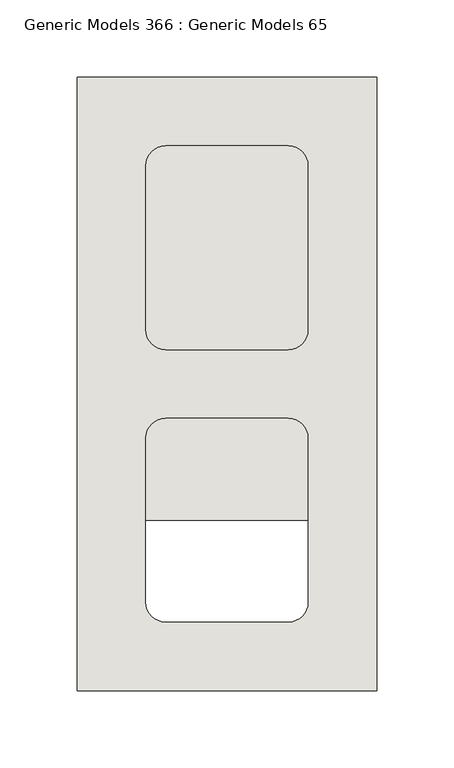
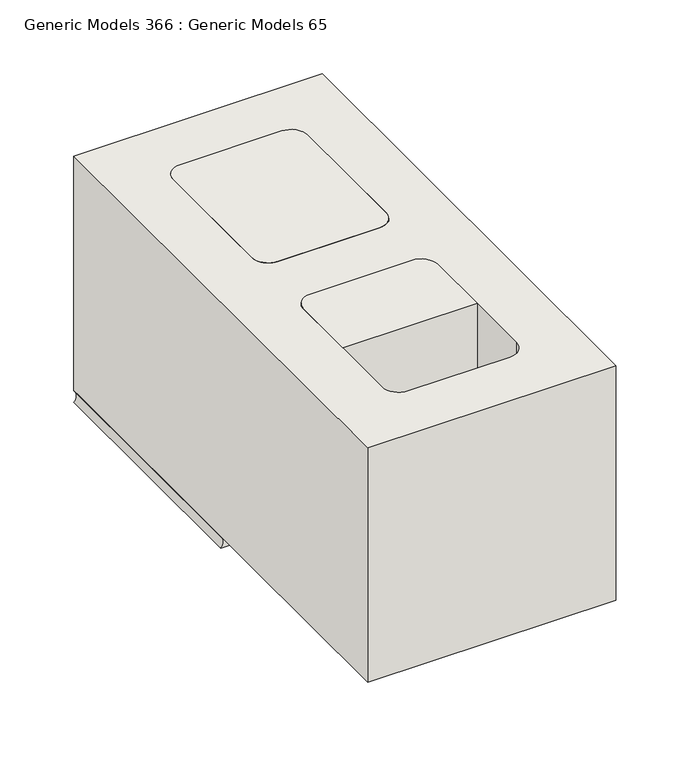
"""IFC4 building model written with IfcOpenShell, lengths in millimetres: wall geometry, Generic Models 366 : Generic Models 65."""

import ifcopenshell
import ifcopenshell.guid

model = None  # the IFC model being written
_history = None  # IfcOwnerHistory: only IFC2X3 demands one
_inside = {}  # id of a spatial element -> (the spatial element, [elements in it])
_under = {}  # id of a project, library or spatial element -> (it, [spatial elements below it])
_declared = {}  # id of a project -> (the project, [libraries it declares])
_typed = {}  # id of a type object -> (the type object, [elements of that type])
_made_of = {}  # id of a material, layer set ... -> (it, [elements and type objects made of it])


def new_model(schema):
    """Start an empty IFC model of exactly this schema.

    Asked for "IFC4X3", IfcOpenShell would pick the latest addendum, in which some entities
    have other attributes; the version numbers below select the first issue.
    IFC2X3 requires an IfcOwnerHistory on every rooted entity: one is made here for all.
    """
    global model, _history
    if schema == "IFC4X3":
        model = ifcopenshell.file(schema_version=(4, 3, 0, 0))
    else:
        model = ifcopenshell.file(schema=schema)
    _inside.clear()
    _under.clear()
    _declared.clear()
    _typed.clear()
    _made_of.clear()
    _history = None
    if model.schema == "IFC2X3":
        org = make("IfcOrganization", Name="unknown")
        user = make(
            "IfcPersonAndOrganization",
            ThePerson=make("IfcPerson", FamilyName="unknown"),
            TheOrganization=org,
        )
        app = make(
            "IfcApplication",
            ApplicationDeveloper=org,
            Version="unknown",
            ApplicationFullName="unknown",
            ApplicationIdentifier="unknown",
        )
        _history = make(
            "IfcOwnerHistory",
            OwningUser=user,
            OwningApplication=app,
            ChangeAction="ADDED",
            CreationDate=0,
        )
    return model


def make(cls, **values):
    """One entity of the class cls with the attributes given. An attribute that is None is left unset."""
    return model.create_entity(
        cls, **{name: value for name, value in values.items() if value is not None}
    )


def rooted(cls, **values):
    """An entity with a GlobalId (a new one), such as an element, a storey or a relation."""
    return make(cls, GlobalId=ifcopenshell.guid.new(), OwnerHistory=_history, **values)


def si_unit(unit_type, name, prefix=None):
    """IfcSIUnit, for example si_unit("LENGTHUNIT", "METRE", prefix="MILLI")."""
    return make("IfcSIUnit", UnitType=unit_type, Prefix=prefix, Name=name)


def assignment(units):
    """IfcUnitAssignment: the units of a project."""
    return None if units is None else make("IfcUnitAssignment", Units=units)


def point(xyz):
    """IfcCartesianPoint."""
    return None if xyz is None else make("IfcCartesianPoint", Coordinates=xyz)


def direction(xyz):
    """IfcDirection."""
    return None if xyz is None else make("IfcDirection", DirectionRatios=xyz)


def frame(location, z_axis=None, x_axis=None):
    """IfcAxis2Placement3D, a coordinate frame: its origin and axes. An axis left out is left unset."""
    return make(
        "IfcAxis2Placement3D",
        Location=point(location),
        Axis=direction(z_axis),
        RefDirection=direction(x_axis),
    )


def frame_2d(location, x_axis=None):
    """IfcAxis2Placement2D, a coordinate frame in the plane: its origin and x axis."""
    return make(
        "IfcAxis2Placement2D", Location=point(location), RefDirection=direction(x_axis)
    )


def origin():
    """The frame at (0, 0, 0) with its axes left unset."""
    return frame((0.0, 0.0, 0.0))


def place(relative_to, where):
    """IfcLocalPlacement: puts the frame where relative to a parent placement (None: the world)."""
    return make(
        "IfcLocalPlacement", PlacementRelTo=relative_to, RelativePlacement=where
    )


def context(
    kind, dimensions, precision=None, world=None, true_north=None, identifier=None
):
    """IfcGeometricRepresentationContext, for example the 3D "Model" context."""
    return make(
        "IfcGeometricRepresentationContext",
        ContextIdentifier=identifier,
        ContextType=kind,
        CoordinateSpaceDimension=dimensions,
        Precision=precision,
        WorldCoordinateSystem=world,
        TrueNorth=true_north,
    )


def project(units=None, contexts=None):
    """IfcProject with its units and contexts."""
    return rooted(
        "IfcProject",
        Name="project",
        RepresentationContexts=contexts,
        UnitsInContext=assignment(units),
    )


def spatial(cls, under=None, at=None, **own):
    """A site, building, storey or space (cls), placed at a placement, below another one or the project."""
    s = rooted(cls, ObjectPlacement=at, **own)
    if under is not None:
        _under.setdefault(under.id(), (under, []))[1].append(s)
    return s


def polyline(points):
    """IfcPolyline through the points."""
    return make("IfcPolyline", Points=[point(p) for p in points])


def circle_curve(where, radius):
    """IfcCircle in the frame where."""
    return make("IfcCircle", Position=where, Radius=radius)


def trimmed(basis, trim1, trim2, sense, master):
    """IfcTrimmedCurve: the piece of a basis curve between two trims."""
    return make(
        "IfcTrimmedCurve",
        BasisCurve=basis,
        Trim1=trim1,
        Trim2=trim2,
        SenseAgreement=sense,
        MasterRepresentation=master,
    )


def segment(curve, same_sense, transition):
    """IfcCompositeCurveSegment."""
    return make(
        "IfcCompositeCurveSegment",
        Transition=transition,
        SameSense=same_sense,
        ParentCurve=curve,
    )


def composite_curve(segments, self_intersect=None):
    """IfcCompositeCurve: segments joined end to end."""
    return make("IfcCompositeCurve", Segments=segments, SelfIntersect=self_intersect)


def outline(outer, holes=None, kind="AREA"):
    """IfcArbitraryClosedProfileDef: a profile drawn as a closed curve; with holes, ...WithVoids."""
    if holes is None:
        return make("IfcArbitraryClosedProfileDef", ProfileType=kind, OuterCurve=outer)
    return make(
        "IfcArbitraryProfileDefWithVoids",
        ProfileType=kind,
        OuterCurve=outer,
        InnerCurves=holes,
    )


def extrude(swept, where, along, depth):
    """IfcExtrudedAreaSolid: the profile swept, set in the frame where, extruded along a direction by depth."""
    return make(
        "IfcExtrudedAreaSolid",
        SweptArea=swept,
        Position=where,
        ExtrudedDirection=direction(along),
        Depth=depth,
    )


def shape(context_of_items, identifier, shape_type, items):
    """IfcShapeRepresentation: the items that make up one representation, for example the "Body"."""
    return make(
        "IfcShapeRepresentation",
        ContextOfItems=context_of_items,
        RepresentationIdentifier=identifier,
        RepresentationType=shape_type,
        Items=items,
    )


def source(mapping_origin, context_of_items, identifier, shape_type, items):
    """IfcRepresentationMap: a shape defined once, which mapped items show again and again."""
    return make(
        "IfcRepresentationMap",
        MappingOrigin=mapping_origin,
        MappedRepresentation=shape(context_of_items, identifier, shape_type, items),
    )


def transform(
    local_origin,
    x_axis=None,
    y_axis=None,
    z_axis=None,
    scale=None,
    scale2=None,
    scale3=None,
    uniform=True,
):
    """IfcCartesianTransformationOperator3D, or its non-uniform kind. x_axis, y_axis, z_axis: its Axis1, 2, 3."""
    if uniform:
        return make(
            "IfcCartesianTransformationOperator3D",
            Axis1=direction(x_axis),
            Axis2=direction(y_axis),
            LocalOrigin=point(local_origin),
            Scale=scale,
            Axis3=direction(z_axis),
        )
    return make(
        "IfcCartesianTransformationOperator3DnonUniform",
        Axis1=direction(x_axis),
        Axis2=direction(y_axis),
        LocalOrigin=point(local_origin),
        Scale=scale,
        Axis3=direction(z_axis),
        Scale2=scale2,
        Scale3=scale3,
    )


def mapped(mapping_source, mapping_target):
    """IfcMappedItem: shows the shape of a source again, moved by a transform."""
    return make(
        "IfcMappedItem", MappingSource=mapping_source, MappingTarget=mapping_target
    )


def made_of(thing, what):
    """Note that an element or type object is made of a material, layer set ...; save() writes the relation."""
    if what is not None:
        _made_of.setdefault(what.id(), (what, []))[1].append(thing)
    return thing


def element(
    cls,
    number,
    at=None,
    inside=None,
    cuts=None,
    type_object=None,
    material=None,
    context=None,
    identifier="Body",
    shape_type=None,
    held_by="IfcProductDefinitionShape",
    body=None,
    shapes=None,
    **own,
):
    """One element of the class cls, such as IfcWall. Its Tag is "e" and its number.

    at: its placement. inside: the storey or other place that contains it. cuts: it is an
    opening in that element (IfcRelVoidsElement). A single representation is given by context,
    identifier, shape_type and body (its items); several are given by shapes. held_by: the class
    of the entity that holds the representations. save() writes the other relations.
    """
    e = rooted(cls, Tag="e%d" % number, ObjectPlacement=at, **own)
    if body is not None:
        shapes = [shape(context, identifier, shape_type, body)]
    if shapes is not None:
        e.Representation = make(held_by, Representations=shapes)
    if inside is not None:
        _inside.setdefault(inside.id(), (inside, []))[1].append(e)
    if cuts is not None:
        rooted(
            "IfcRelVoidsElement", RelatingBuildingElement=cuts, RelatedOpeningElement=e
        )
    if type_object is not None:
        _typed.setdefault(type_object.id(), (type_object, []))[1].append(e)
    return made_of(e, material)


def aggregate(whole, parts):
    """IfcRelAggregates: a whole, such as a stair, and the parts it consists of."""
    return rooted("IfcRelAggregates", RelatingObject=whole, RelatedObjects=parts)


def save(model, path):
    """Write the relations noted so far, then the file.

    IfcRelAggregates (storeys below a building ...), IfcRelContainedInSpatialStructure (elements
    in a storey), IfcRelDefinesByType, IfcRelAssociatesMaterial and IfcRelDeclares: one each for
    every whole, place, type object, material and project.
    """
    for whole, parts in _under.values():
        aggregate(whole, parts)
    for where, things in _inside.values():
        rooted(
            "IfcRelContainedInSpatialStructure",
            RelatedElements=things,
            RelatingStructure=where,
        )
    for kind, things in _typed.values():
        rooted("IfcRelDefinesByType", RelatedObjects=things, RelatingType=kind)
    for what, things in _made_of.values():
        rooted("IfcRelAssociatesMaterial", RelatedObjects=things, RelatingMaterial=what)
    for by, libraries in _declared.values():
        rooted("IfcRelDeclares", RelatingContext=by, RelatedDefinitions=libraries)
    model.write(path)


def plane_surface(at):
    """IfcPlane: the flat surface through the origin of the frame at, square to its z axis."""
    return make("IfcPlane", Position=at)


def revolved_surface(curve, axis_point, axis_direction):
    """IfcSurfaceOfRevolution: the curve turned about the line through axis_point along axis_direction."""
    return make(
        "IfcSurfaceOfRevolution",
        SweptCurve=make("IfcArbitraryOpenProfileDef", ProfileType="CURVE", Curve=curve),
        AxisPosition=make("IfcAxis1Placement", Location=point(axis_point), Axis=direction(axis_direction)),
    )


def advanced_brep(points, edges, surfaces, faces):
    """IfcAdvancedBrep: a solid bounded by faces that lie on surfaces and meet in shared edges.

    An edge is (start, end): straight between two places in points (the first is 0);
    or (start, end, curve); or (start, end, curve, False) where it runs against its curve.
    A face is (place in surfaces, loops), or (place, loops, False) where it looks against
    its surface's normal. A loop lists edges by number (the first is 1), with a minus sign
    where the edge is run from its end to its start. The first loop is the outer one.
    """
    corners = [point(p) for p in points]
    vertices = [make("IfcVertexPoint", VertexGeometry=c) for c in corners]
    made = []
    for start, end, *more in edges:
        made.append(
            make(
                "IfcEdgeCurve",
                EdgeStart=vertices[start],
                EdgeEnd=vertices[end],
                EdgeGeometry=more[0] if more else make("IfcPolyline", Points=[corners[start], corners[end]]),
                SameSense=more[1] if len(more) > 1 else True,
            )
        )
    hull = []
    for where, loops, *sense in faces:
        bounds = []
        for j, loop in enumerate(loops):
            ring = [make("IfcOrientedEdge", EdgeElement=made[abs(k) - 1], Orientation=k > 0) for k in loop]
            bounds.append(
                make(
                    "IfcFaceOuterBound" if j == 0 else "IfcFaceBound",
                    Bound=make("IfcEdgeLoop", EdgeList=ring),
                    Orientation=True,
                )
            )
        hull.append(make("IfcAdvancedFace", Bounds=bounds, FaceSurface=surfaces[where], SameSense=sense[0] if sense else True))
    return make("IfcAdvancedBrep", Outer=make("IfcClosedShell", CfsFaces=hull))


def generic_models_366_generic_models_65_ef9577f4(model_context):
    return source(origin(), model_context, "Body", "SolidModel", [
        advanced_brep(
        [(430198.2125, 503.2375, 1635.125), (430004.5375, 503.2375, 1635.125), (430004.5375, 503.2375, 1625.6), (430198.2125, 503.2375, 1625.6), (430198.2125, 701.675, 1635.125), (430198.2125, 701.675, 1625.6), (430004.5375, 701.675, 1625.6), (430004.5375, 701.675, 1635.125), (430153.7625, 538.1625, 1635.125), (430141.0625, 525.4625, 1635.125), (430061.6875, 525.4625, 1635.125), (430048.9875, 538.1625, 1635.125), (430048.9875, 644.525, 1635.125), (430061.6875, 657.225, 1635.125), (430141.0625, 657.225, 1635.125), (430153.7625, 644.525, 1635.125), (430141.0625, 525.4625, 1625.6), (430153.7625, 538.1625, 1625.6), (430061.6875, 525.4625, 1625.6), (430048.9875, 538.1625, 1625.6), (430048.9875, 644.525, 1625.6), (430061.6875, 657.225, 1625.6), (430141.0625, 657.225, 1625.6), (430153.7625, 644.525, 1625.6)],
        [
            (0, 1),
            (1, 2, circle_curve(frame((429999.6545028, 503.2375, 1630.3625), z_axis=(0.0, 1.0, 0.0), x_axis=(1.0, 0.0, 0.0)), 6.8209287)),
            (2, 3),
            (3, 0, circle_curve(frame((430203.0954972, 503.2375, 1630.3625), z_axis=(0.0, 1.0, 0.0), x_axis=(-1.0, 0.0, 0.0)), 6.8209287)),
            (4, 5, circle_curve(frame((430203.0954972, 701.675, 1630.3625), z_axis=(0.0, -1.0, 0.0), x_axis=(-1.0, 0.0, 0.0)), 6.8209287)),
            (5, 6),
            (6, 7, circle_curve(frame((429999.6545028, 701.675, 1630.3625), z_axis=(0.0, -1.0, 0.0), x_axis=(1.0, 0.0, 0.0)), 6.8209287)),
            (7, 4),
            (0, 4),
            (7, 1),
            (8, 9, circle_curve(frame((430141.0625, 538.1625, 1635.125), z_axis=(0.0, 0.0, -1.0), x_axis=(-1.0, 0.0, 0.0)), 12.7)),
            (9, 10),
            (10, 11, circle_curve(frame((430061.6875, 538.1625, 1635.125), z_axis=(0.0, 0.0, -1.0), x_axis=(-1.0, 0.0, 0.0)), 12.7)),
            (11, 12),
            (12, 13, circle_curve(frame((430061.6875, 644.525, 1635.125), z_axis=(0.0, 0.0, -1.0), x_axis=(-1.0, 0.0, 0.0)), 12.7)),
            (13, 14),
            (14, 15, circle_curve(frame((430141.0625, 644.525, 1635.125), z_axis=(0.0, 0.0, -1.0), x_axis=(-1.0, 0.0, 0.0)), 12.7)),
            (15, 8),
            (16, 9),
            (8, 17),
            (17, 16, circle_curve(frame((430141.0625, 538.1625, 1625.6), z_axis=(0.0, 0.0, -1.0), x_axis=(-1.0, 0.0, 0.0)), 12.7)),
            (16, 18),
            (18, 10),
            (18, 19, circle_curve(frame((430061.6875, 538.1625, 1625.6), z_axis=(0.0, 0.0, -1.0), x_axis=(-1.0, 0.0, 0.0)), 12.7)),
            (19, 11),
            (19, 20),
            (20, 12),
            (20, 21, circle_curve(frame((430061.6875, 644.525, 1625.6), z_axis=(0.0, 0.0, -1.0), x_axis=(-1.0, 0.0, 0.0)), 12.7)),
            (21, 13),
            (21, 22),
            (22, 14),
            (22, 23, circle_curve(frame((430141.0625, 644.525, 1625.6), z_axis=(0.0, 0.0, -1.0), x_axis=(-1.0, 0.0, 0.0)), 12.7)),
            (23, 15),
            (23, 17),
            (6, 2),
            (5, 3),
        ],
        [
            plane_surface(frame((430101.375, 503.2375, 1635.521875), z_axis=(0.0, -1.0, 0.0), x_axis=(0.0, 0.0, 1.0))),
            plane_surface(frame((430101.375, 701.675, 1635.521875), z_axis=(0.0, 1.0, 0.0), x_axis=(0.0, 0.0, 1.0))),
            plane_surface(frame((430198.2125, 503.2375, 1635.125), z_axis=(0.0, 0.0, 1.0), x_axis=(0.0, 1.0, 0.0))),
            revolved_surface(polyline([(430128.3625, 538.1625, 1635.125), (430128.3625, 538.1625, 1625.6)]), (430141.0625, 538.1625, 1819.275), (0.0, 0.0, 1.0)),
            plane_surface(frame((430061.6875, 525.4625, 1819.275), z_axis=(0.0, 1.0, 0.0), x_axis=(0.0, 0.0, -1.0))),
            revolved_surface(polyline([(430048.9875, 538.1625, 1635.125), (430048.9875, 538.1625, 1625.6)]), (430061.6875, 538.1625, 1819.275), (0.0, 0.0, 1.0)),
            plane_surface(frame((430048.9875, 644.525, 1819.275), z_axis=(1.0, 0.0, 0.0), x_axis=(0.0, 0.0, -1.0))),
            revolved_surface(polyline([(430048.9875, 644.525, 1635.125), (430048.9875, 644.525, 1625.6)]), (430061.6875, 644.525, 1819.275), (0.0, 0.0, 1.0)),
            plane_surface(frame((430141.0625, 657.225, 1819.275), z_axis=(0.0, -1.0, 0.0), x_axis=(0.0, 0.0, -1.0))),
            revolved_surface(polyline([(430128.3625, 644.525, 1635.125), (430128.3625, 644.525, 1625.6)]), (430141.0625, 644.525, 1819.275), (0.0, 0.0, 1.0)),
            plane_surface(frame((430153.7625, 538.1625, 1819.275), z_axis=(-1.0, 0.0, 0.0), x_axis=(0.0, 0.0, -1.0))),
            revolved_surface(polyline([(430006.4754315, 701.675, 1630.3625), (430006.4754315, 503.2375, 1630.3625)]), (429999.6545028, 503.2375, 1630.3625), (0.0, 1.0, 0.0)),
            plane_surface(frame((430004.5375, 503.2375, 1625.6), z_axis=(0.0, 0.0, -1.0), x_axis=(0.0, 1.0, 0.0))),
            revolved_surface(polyline([(430196.2745685, 701.675, 1630.3625), (430196.2745685, 503.2375, 1630.3625)]), (430203.0954972, 503.2375, 1630.3625), (0.0, 1.0, 0.0)),
        ],
        [
            (0, [[1, 2, 3, 4]]),
            (1, [[5, 6, 7, 8]]),
            (2, [[-1, 9, -8, 10], [11, 12, 13, 14, 15, 16, 17, 18]]),
            (3, [[19, -11, 20, 21]]),
            (4, [[-19, 22, 23, -12]]),
            (5, [[-23, 24, 25, -13]]),
            (6, [[-25, 26, 27, -14]]),
            (7, [[-27, 28, 29, -15]]),
            (8, [[-29, 30, 31, -16]]),
            (9, [[-31, 32, 33, -17]]),
            (10, [[-33, 34, -20, -18]]),
            (11, [[-2, -10, -7, 35]]),
            (12, [[-3, -35, -6, 36], [-21, -34, -32, -30, -28, -26, -24, -22]]),
            (13, [[-4, -36, -5, -9]]),
        ],
    ),
        extrude(outline(composite_curve([segment(trimmed(circle_curve(frame_2d((430141.0625, 538.1625)), 12.7), [point((430153.7625, 538.1625))], [point((430141.0625, 525.4625))], False, "CARTESIAN"), True, "CONTINUOUS"), segment(polyline([(430141.0625, 525.4625), (430061.6875, 525.4625)]), True, "CONTINUOUS"), segment(trimmed(circle_curve(frame_2d((430061.6875, 538.1625)), 12.7), [point((430061.6875, 525.4625))], [point((430048.9875, 538.1625))], False, "CARTESIAN"), True, "CONTINUOUS"), segment(polyline([(430048.9875, 538.1625), (430048.9875, 644.525)]), True, "CONTINUOUS"), segment(trimmed(circle_curve(frame_2d((430061.6875, 644.525)), 12.7), [point((430048.9875, 644.525))], [point((430061.6875, 657.225))], False, "CARTESIAN"), True, "CONTINUOUS"), segment(polyline([(430061.6875, 657.225), (430141.0625, 657.225)]), True, "CONTINUOUS"), segment(trimmed(circle_curve(frame_2d((430141.0625, 644.525)), 12.7), [point((430141.0625, 657.225))], [point((430153.7625, 644.525))], False, "CARTESIAN"), True, "CONTINUOUS"), segment(polyline([(430153.7625, 644.525), (430153.7625, 538.1625)]), True, "CONTINUOUS")], self_intersect=False)), frame((0.0, 0.0, 1625.6), z_axis=(0.0, 0.0, 1.0), x_axis=(1.0, 0.0, 0.0)), (0.0, 0.0, 1.0), 203.2),
        extrude(outline(composite_curve([segment(trimmed(circle_curve(frame_2d((430061.6875, 468.3125)), 12.7), [point((430048.9875, 468.3125))], [point((430061.6875, 481.0125))], False, "CARTESIAN"), True, "CONTINUOUS"), segment(polyline([(430061.6875, 481.0125), (430141.0625, 481.0125)]), True, "CONTINUOUS"), segment(trimmed(circle_curve(frame_2d((430141.0625, 468.3125)), 12.7), [point((430141.0625, 481.0125))], [point((430153.7625, 468.3125))], False, "CARTESIAN"), True, "CONTINUOUS"), segment(polyline([(430153.7625, 468.3125), (430153.7625, 415.13125), (430048.9875, 415.13125), (430048.9875, 468.3125)]), True, "CONTINUOUS")], self_intersect=False)), frame((0.0, 0.0, 1625.6), z_axis=(0.0, 0.0, 1.0), x_axis=(1.0, 0.0, 0.0)), (0.0, 0.0, 1.0), 203.2),
        extrude(outline(polyline([(430198.2125, 304.8), (430004.5375, 304.8), (430004.5375, 701.675), (430198.2125, 701.675), (430198.2125, 304.8)]), holes=[composite_curve([segment(polyline([(430153.7625, 538.1625), (430153.7625, 644.525)]), True, "CONTINUOUS"), segment(trimmed(circle_curve(frame_2d((430141.0625, 644.525)), 12.7), [point((430153.7625, 644.525))], [point((430141.0625, 657.225))], True, "CARTESIAN"), True, "CONTINUOUS"), segment(polyline([(430141.0625, 657.225), (430061.6875, 657.225)]), True, "CONTINUOUS"), segment(trimmed(circle_curve(frame_2d((430061.6875, 644.525)), 12.7), [point((430061.6875, 657.225))], [point((430048.9875, 644.525))], True, "CARTESIAN"), True, "CONTINUOUS"), segment(polyline([(430048.9875, 644.525), (430048.9875, 538.1625)]), True, "CONTINUOUS"), segment(trimmed(circle_curve(frame_2d((430061.6875, 538.1625)), 12.7), [point((430048.9875, 538.1625))], [point((430061.6875, 525.4625))], True, "CARTESIAN"), True, "CONTINUOUS"), segment(polyline([(430061.6875, 525.4625), (430141.0625, 525.4625)]), True, "CONTINUOUS"), segment(trimmed(circle_curve(frame_2d((430141.0625, 538.1625)), 12.7), [point((430141.0625, 525.4625))], [point((430153.7625, 538.1625))], True, "CARTESIAN"), True, "CONTINUOUS")], self_intersect=False), composite_curve([segment(polyline([(430048.9875, 468.3125), (430048.9875, 361.95)]), True, "CONTINUOUS"), segment(trimmed(circle_curve(frame_2d((430061.6875, 361.95)), 12.7), [point((430048.9875, 361.95))], [point((430061.6875, 349.25))], True, "CARTESIAN"), True, "CONTINUOUS"), segment(polyline([(430061.6875, 349.25), (430141.0625, 349.25)]), True, "CONTINUOUS"), segment(trimmed(circle_curve(frame_2d((430141.0625, 361.95)), 12.7), [point((430141.0625, 349.25))], [point((430153.7625, 361.95))], True, "CARTESIAN"), True, "CONTINUOUS"), segment(polyline([(430153.7625, 361.95), (430153.7625, 468.3125)]), True, "CONTINUOUS"), segment(trimmed(circle_curve(frame_2d((430141.0625, 468.3125)), 12.7), [point((430153.7625, 468.3125))], [point((430141.0625, 481.0125))], True, "CARTESIAN"), True, "CONTINUOUS"), segment(polyline([(430141.0625, 481.0125), (430061.6875, 481.0125)]), True, "CONTINUOUS"), segment(trimmed(circle_curve(frame_2d((430061.6875, 468.3125)), 12.7), [point((430061.6875, 481.0125))], [point((430048.9875, 468.3125))], True, "CARTESIAN"), True, "CONTINUOUS")], self_intersect=False)]), frame((0.0, 0.0, 1635.125), z_axis=(0.0, 0.0, 1.0), x_axis=(1.0, 0.0, 0.0)), (0.0, 0.0, 1.0), 193.675),
    ])


if __name__ == "__main__":
    model = new_model("IFC4")
    model_context = context("Model", 3, world=origin())
    ifc_project = project(units=[si_unit("LENGTHUNIT", "METRE", prefix="MILLI")], contexts=[model_context])
    site = spatial("IfcSite", under=ifc_project)
    building = spatial("IfcBuilding", under=site)
    placement = place(None, origin())
    generic_models_366_generic_models_65_shape = generic_models_366_generic_models_65_ef9577f4(model_context)
    element("IfcWall", 1, ObjectType="Generic Models 366 : Generic Models 65", at=placement, inside=building, context=model_context, shape_type="MappedRepresentation", body=[
        mapped(generic_models_366_generic_models_65_shape, transform((0.0, 0.0, 0.0), x_axis=(1.0, 0.0, 0.0), y_axis=(0.0, 1.0, 0.0), z_axis=(0.0, 0.0, 1.0))),
    ])
    save(model, "model.ifc")

# Revit data of these elements
# Element 1 (IfcWall, "Generic Models 366 : Generic Models 65")
#   Materials on its faces: "CMU (SEE 'WALL TAG' FOR SIZE)", "FILL CORE IF APPLICABLE - SEE STRUCTURAL DWGS FOR DETAILS", "MORTAR JOINT"
# Materials
#   "CMU (SEE 'WALL TAG' FOR SIZE)": class "Masonry", colour RGB 203 203 199, transparency 0, Description = "Concrete masonry units", Cost = 0
#   "FILL CORE IF APPLICABLE - SEE STRUCTURAL DWGS FOR DETAILS": class "Generic", colour RGB 170 170 170, transparency 0, Cost = 0
#   "MORTAR JOINT": class "Generic", colour RGB 120 120 120, transparency 0, Cost = 0
